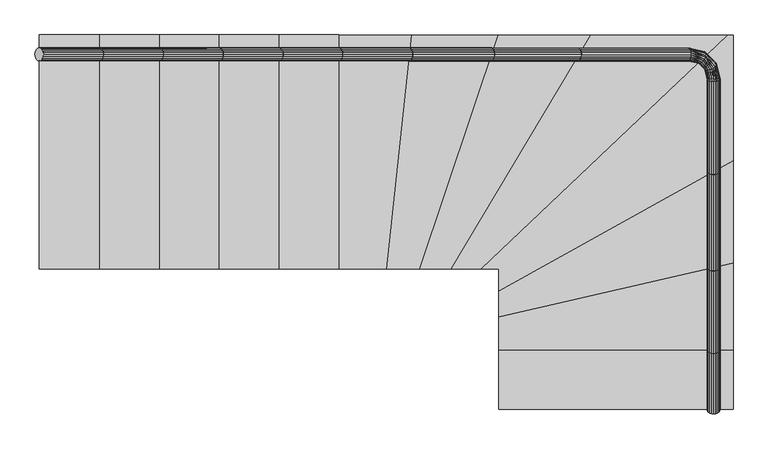
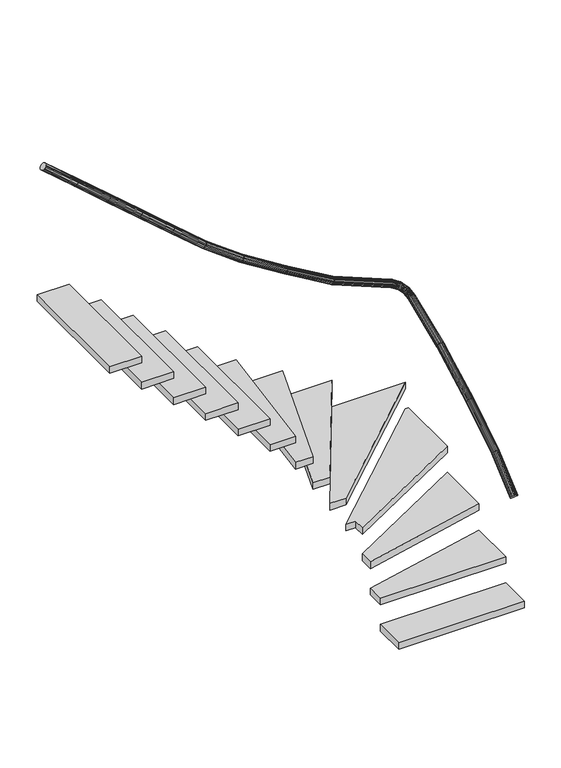
"""IFC4 building model written with IfcOpenShell, lengths in millimetres: stair geometry, 0_3d_modell."""

from ifc_helpers import new_model, si_unit, frame, origin, origin_with_axes, place, context, project, spatial, polyline, outline, extrude, faceted_brep, source, transform, mapped, element, save


def stair_9e6d9002(model_context):
    return source(origin(), model_context, "Body", "SolidModel", [
        extrude(outline(polyline([(1781.5036957, 473.824936), (1781.5036957, 556.9018591), (1711.5036957, 556.9018591), (2658.8332796, 1456.9018591), (2681.5036957, 1456.9018591), (2681.5036957, 973.1970565), (1781.5036957, 473.824936)])), frame((0.0, 0.0, 595.7142857), z_axis=(0.0, 0.0, 1.0), x_axis=(1.0, 0.0, 0.0)), (0.0, 0.0, 1.0), 50.0),
        extrude(outline(polyline([(936.9018591, 556.9018591), (706.9018591, 556.9018591), (706.9018591, 1456.9018591), (936.9018591, 1456.9018591), (936.9018591, 556.9018591)])), frame((0.0, 0.0, 1787.1428571), z_axis=(0.0, 0.0, 1.0), x_axis=(1.0, 0.0, 0.0)), (0.0, 0.0, 1.0), 50.0),
        extrude(outline(polyline([(1.2235871, -7.9923214), (0.0, 0.0), (1.2235871, 7.9923214), (4.7745751, 15.2022987), (10.3053687, 20.9241691), (17.2745751, 24.597836), (25.0, 25.8636953), (32.7254248, 24.597836), (39.6946313, 20.9241691), (45.2254248, 15.2022987), (48.7764129, 7.9923214), (50.0, 0.0), (48.7764129, -7.9923214), (45.2254248, -15.2022986), (39.6946313, -20.9241689), (32.7254248, -24.5978359), (25.0, -25.8636953), (17.2745751, -24.5978359), (10.3053687, -20.9241689), (4.7745751, -15.2022986), (1.2235871, -7.9923214)])), frame((936.9018591, 1406.9018591, 2656.7020937), z_axis=(-0.7569287102857389, 0.0, 0.6534974579485127), x_axis=(0.0, -1.0, 0.0)), (0.0, 0.0, 1.0), 303.8595272),
        extrude(outline(polyline([(1349.1921789, 556.9018591), (1166.9018591, 556.9018591), (1166.9018591, 1456.9018591), (1444.6115394, 1456.9018591), (1349.1921789, 556.9018591)])), frame((0.0, 0.0, 1390.0), z_axis=(0.0, 0.0, 1.0), x_axis=(1.0, 0.0, 0.0)), (0.0, 0.0, 1.0), 50.0),
        extrude(outline(polyline([(1477.0220692, 556.9018591), (1349.1921789, 556.9018591), (1444.6115394, 1456.9018591), (1776.781649, 1456.9018591), (1477.0220692, 556.9018591)])), frame((0.0, 0.0, 1191.4285714), z_axis=(0.0, 0.0, 1.0), x_axis=(1.0, 0.0, 0.0)), (0.0, 0.0, 1.0), 50.0),
        extrude(outline(polyline([(1711.5036957, 556.9018591), (1597.1723093, 556.9018591), (2132.6233472, 1456.9018591), (2658.8332796, 1456.9018591), (1711.5036957, 556.9018591)])), frame((0.0, 0.0, 794.2857143), z_axis=(0.0, 0.0, 1.0), x_axis=(1.0, 0.0, 0.0)), (0.0, 0.0, 1.0), 50.0),
        extrude(outline(polyline([(1.2235871, -7.9923214), (0.0, 0.0), (1.2235871, 7.9923214), (4.7745751, 15.2022986), (10.3053687, 20.924169), (17.2745751, 24.5978359), (25.0, 25.8636953), (32.7254248, 24.5978359), (39.6946313, 20.924169), (45.2254248, 15.2022986), (48.7764129, 7.9923214), (50.0, 0.0), (48.7764129, -7.9923214), (45.2254248, -15.2022986), (39.6946313, -20.924169), (32.7254248, -24.597836), (25.0, -25.8636953), (17.2745751, -24.597836), (10.3053687, -20.924169), (4.7745751, -15.2022986), (1.2235871, -7.9923214)])), frame((246.9018591, 1406.9018591, 3252.4163795), z_axis=(-0.7569287102857456, 0.0, 0.6534974579485049), x_axis=(0.0, -1.0, 0.0)), (0.0, 0.0, 1.0), 303.8595272),
        faceted_brep([(2630.2801086, 935.0213576, 1458.0478269), (2631.5036957, 931.5827131, 1465.2735223), (2630.2801086, 928.1440687, 1472.4992177), (2626.7291206, 925.0420228, 1479.0176117), (2621.198327, 922.5802252, 1484.1906384), (2614.2291206, 920.9996538, 1487.511926), (2606.5036957, 920.4550261, 1488.6563638), (2598.7782709, 920.9996538, 1487.511926), (2591.8090644, 922.5802252, 1484.1906384), (2586.2782709, 925.0420228, 1479.0176117), (2582.7272828, 928.1440687, 1472.4992177), (2581.5036957, 931.5827131, 1465.2735223), (2582.7272828, 935.0213576, 1458.0478269), (2586.2782709, 938.1234035, 1451.529433), (2591.8090644, 940.5852011, 1446.3564062), (2598.7782709, 942.1657724, 1443.0351186), (2606.5036957, 942.7104002, 1441.8906809), (2614.2291206, 942.1657724, 1443.0351186), (2621.198327, 940.5852011, 1446.3564062), (2626.7291206, 938.1234035, 1451.529433), (2630.2801086, 1283.3224302, 1620.3777918), (2631.5036957, 1286.3944101, 1612.9994356), (2630.2801086, 1289.46639, 1605.6210794), (2626.7291206, 1292.2376632, 1598.9649681), (2621.198327, 1294.436958, 1593.6826483), (2614.2291206, 1295.8489921, 1590.2911902), (2606.5036957, 1296.335546, 1589.1225734), (2598.7782709, 1295.8489921, 1590.2911902), (2591.8090644, 1294.436958, 1593.6826483), (2586.2782709, 1292.2376632, 1598.9649681), (2582.7272828, 1289.46639, 1605.6210794), (2581.5036957, 1286.3944101, 1612.9994356), (2582.7272828, 1283.3224302, 1620.3777918), (2586.2782709, 1280.5511571, 1627.0339031), (2591.8090644, 1278.3518623, 1632.3162229), (2598.7782709, 1276.9398281, 1635.707681), (2606.5036957, 1276.4532743, 1636.8762979), (2614.2291206, 1276.9398281, 1635.707681), (2621.198327, 1278.3518623, 1632.3162229), (2626.7291206, 1280.5511571, 1627.0339031)], [[[0, 1, 2, 3, 4, 5, 6, 7, 8, 9, 10, 11, 12, 13, 14, 15, 16, 17, 18, 19]], [[20, 21, 22, 23, 24, 25, 26, 27, 28, 29, 30, 31, 32, 33, 34, 35, 36, 37, 38, 39]], [[2, 1, 21, 20]], [[3, 2, 20, 39]], [[4, 3, 39, 38]], [[5, 4, 38, 37]], [[6, 5, 37, 36]], [[7, 6, 36, 35]], [[8, 7, 35, 34]], [[9, 8, 34, 33]], [[10, 9, 33, 32]], [[11, 10, 32, 31]], [[12, 11, 31, 30]], [[13, 12, 30, 29]], [[14, 13, 29, 28]], [[15, 14, 28, 27]], [[16, 15, 27, 26]], [[17, 16, 26, 25]], [[18, 17, 25, 24]], [[19, 18, 24, 23]], [[0, 19, 23, 22]], [[1, 0, 22, 21]]]),
        extrude(outline(polyline([(1781.5036957, 373.9346688), (1781.5036957, 473.824936), (2681.5036957, 973.1970565), (2681.5036957, 579.8690495), (1781.5036957, 373.9346688)])), frame((0.0, 0.0, 397.1428571), z_axis=(0.0, 0.0, 1.0), x_axis=(1.0, 0.0, 0.0)), (0.0, 0.0, 1.0), 50.0),
        extrude(outline(polyline([(1.2235871, -7.9923214), (0.0, 0.0), (1.2235871, 7.9923214), (4.7745751, 15.2022986), (10.3053687, 20.9241691), (17.2745751, 24.5978359), (25.0, 25.8636953), (32.7254248, 24.5978359), (39.6946313, 20.9241691), (45.2254248, 15.2022986), (48.7764129, 7.9923214), (50.0, 0.0), (48.7764129, -7.9923214), (45.2254248, -15.2022986), (39.6946313, -20.924169), (32.7254248, -24.5978359), (25.0, -25.8636953), (17.2745751, -24.5978359), (10.3053687, -20.924169), (4.7745751, -15.2022986), (1.2235871, -7.9923214)])), frame((476.9018591, 1406.9018591, 3053.8449509), z_axis=(-0.7569287102857636, 0.0, 0.6534974579484839), x_axis=(0.0, -1.0, 0.0)), (0.0, 0.0, 1.0), 303.8595272),
        faceted_brep([(2630.2801086, 566.7337566, 1259.7925307), (2631.5036957, 562.7078511, 1266.7020937), (2630.2801086, 558.6819455, 1273.6116568), (2626.7291206, 555.0501237, 1279.8448636), (2621.198327, 552.1678935, 1284.7915646), (2614.2291206, 550.3173878, 1287.9675421), (2606.5036957, 549.679747, 1289.0619094), (2598.7782709, 550.3173878, 1287.9675421), (2591.8090644, 552.1678935, 1284.7915646), (2586.2782709, 555.0501237, 1279.8448636), (2582.7272828, 558.6819455, 1273.6116568), (2581.5036957, 562.7078511, 1266.7020937), (2582.7272828, 566.7337566, 1259.7925307), (2586.2782709, 570.3655785, 1253.5593239), (2591.8090644, 573.2478087, 1248.6126229), (2598.7782709, 575.0983143, 1245.4366454), (2606.5036957, 575.7359551, 1244.3422781), (2614.2291206, 575.0983143, 1245.4366454), (2621.198327, 573.2478087, 1248.6126229), (2626.7291206, 570.3655785, 1253.5593239), (2630.2801086, 928.1440687, 1472.4992177), (2631.5036957, 931.5827131, 1465.2735223), (2630.2801086, 935.0213576, 1458.0478269), (2626.7291206, 938.1234035, 1451.529433), (2621.198327, 940.5852011, 1446.3564062), (2614.2291206, 942.1657724, 1443.0351186), (2606.5036957, 942.7104002, 1441.8906809), (2598.7782709, 942.1657724, 1443.0351186), (2591.8090644, 940.5852011, 1446.3564062), (2586.2782709, 938.1234035, 1451.529433), (2582.7272828, 935.0213576, 1458.0478269), (2581.5036957, 931.5827131, 1465.2735223), (2582.7272828, 928.1440687, 1472.4992177), (2586.2782709, 925.0420228, 1479.0176117), (2591.8090644, 922.5802252, 1484.1906384), (2598.7782709, 920.9996538, 1487.511926), (2606.5036957, 920.4550261, 1488.6563638), (2614.2291206, 920.9996538, 1487.511926), (2621.198327, 922.5802252, 1484.1906384), (2626.7291206, 925.0420228, 1479.0176117)], [[[0, 1, 2, 3, 4, 5, 6, 7, 8, 9, 10, 11, 12, 13, 14, 15, 16, 17, 18, 19]], [[20, 21, 22, 23, 24, 25, 26, 27, 28, 29, 30, 31, 32, 33, 34, 35, 36, 37, 38, 39]], [[2, 1, 21, 20]], [[3, 2, 20, 39]], [[4, 3, 39, 38]], [[5, 4, 38, 37]], [[6, 5, 37, 36]], [[7, 6, 36, 35]], [[8, 7, 35, 34]], [[9, 8, 34, 33]], [[10, 9, 33, 32]], [[11, 10, 32, 31]], [[12, 11, 31, 30]], [[13, 12, 30, 29]], [[14, 13, 29, 28]], [[15, 14, 28, 27]], [[16, 15, 27, 26]], [[17, 16, 26, 25]], [[18, 17, 25, 24]], [[19, 18, 24, 23]], [[0, 19, 23, 22]], [[1, 0, 22, 21]]]),
        faceted_brep([(2630.2801086, 251.6675536, 1061.6862641), (2631.5036957, 246.9018591, 1068.1306652), (2630.2801086, 242.1361647, 1074.5750662), (2626.7291206, 237.8369696, 1080.3886444), (2621.198327, 234.4251091, 1085.0023262), (2614.2291206, 232.2345598, 1087.9644922), (2606.5036957, 231.4797479, 1088.985185), (2598.7782709, 232.2345598, 1087.9644922), (2591.8090644, 234.4251091, 1085.0023262), (2586.2782709, 237.8369696, 1080.3886444), (2582.7272828, 242.1361647, 1074.5750662), (2581.5036957, 246.9018591, 1068.1306652), (2582.7272828, 251.6675536, 1061.6862641), (2586.2782709, 255.9667486, 1055.872686), (2591.8090644, 259.3786091, 1051.2590042), (2598.7782709, 261.5691584, 1048.2968382), (2606.5036957, 262.3239703, 1047.2761453), (2614.2291206, 261.5691584, 1048.2968382), (2621.198327, 259.3786091, 1051.2590042), (2626.7291206, 255.9667486, 1055.872686), (2630.2801086, 558.6819455, 1273.6116568), (2631.5036957, 562.7078511, 1266.7020937), (2630.2801086, 566.7337566, 1259.7925307), (2626.7291206, 570.3655785, 1253.5593239), (2621.198327, 573.2478087, 1248.6126229), (2614.2291206, 575.0983143, 1245.4366454), (2606.5036957, 575.7359551, 1244.3422781), (2598.7782709, 575.0983143, 1245.4366454), (2591.8090644, 573.2478087, 1248.6126229), (2586.2782709, 570.3655785, 1253.5593239), (2582.7272828, 566.7337566, 1259.7925307), (2581.5036957, 562.7078511, 1266.7020937), (2582.7272828, 558.6819455, 1273.6116568), (2586.2782709, 555.0501237, 1279.8448636), (2591.8090644, 552.1678935, 1284.7915646), (2598.7782709, 550.3173878, 1287.9675421), (2606.5036957, 549.679747, 1289.0619094), (2614.2291206, 550.3173878, 1287.9675421), (2621.198327, 552.1678935, 1284.7915646), (2626.7291206, 555.0501237, 1279.8448636)], [[[0, 1, 2, 3, 4, 5, 6, 7, 8, 9, 10, 11, 12, 13, 14, 15, 16, 17, 18, 19]], [[20, 21, 22, 23, 24, 25, 26, 27, 28, 29, 30, 31, 32, 33, 34, 35, 36, 37, 38, 39]], [[2, 1, 21, 20]], [[3, 2, 20, 39]], [[4, 3, 39, 38]], [[5, 4, 38, 37]], [[6, 5, 37, 36]], [[7, 6, 36, 35]], [[8, 7, 35, 34]], [[9, 8, 34, 33]], [[10, 9, 33, 32]], [[11, 10, 32, 31]], [[12, 11, 31, 30]], [[13, 12, 30, 29]], [[14, 13, 29, 28]], [[15, 14, 28, 27]], [[16, 15, 27, 26]], [[17, 16, 26, 25]], [[18, 17, 25, 24]], [[19, 18, 24, 23]], [[0, 19, 23, 22]], [[1, 0, 22, 21]]]),
        faceted_brep([(2630.2801086, 1289.46639, 1605.6210794), (2631.5036957, 1286.3944101, 1612.9994356), (2630.2801086, 1283.3224302, 1620.3777918), (2626.7291206, 1280.5511571, 1627.0339031), (2621.198327, 1278.3518623, 1632.3162229), (2614.2291206, 1276.9398281, 1635.707681), (2606.5036957, 1276.4532743, 1636.8762979), (2598.7782709, 1276.9398281, 1635.707681), (2591.8090644, 1278.3518623, 1632.3162229), (2586.2782709, 1280.5511571, 1627.0339031), (2582.7272828, 1283.3224302, 1620.3777918), (2581.5036957, 1286.3944101, 1612.9994356), (2582.7272828, 1289.46639, 1605.6210794), (2586.2782709, 1292.2376632, 1598.9649681), (2591.8090644, 1294.436958, 1593.6826483), (2598.7782709, 1295.8489921, 1590.2911902), (2606.5036957, 1296.335546, 1589.1225734), (2614.2291206, 1295.8489921, 1590.2911902), (2621.198327, 1294.436958, 1593.6826483), (2626.7291206, 1292.2376632, 1598.9649681), (2616.4980036, 1348.8501513, 1638.9123688), (2617.3046378, 1344.8271855, 1645.879395), (2615.8855438, 1340.0232633, 1652.1644401), (2612.3796323, 1334.9086261, 1657.1522801), (2607.1300863, 1329.9839302, 1660.3546705), (2600.650768, 1325.7312391, 1661.4581391), (2593.5759183, 1322.5668359, 1660.3546705), (2586.5980727, 1320.8004745, 1657.1522801), (2580.4002713, 1320.6050585, 1652.1644401), (2575.5891981, 1321.9997167, 1645.879395), (2572.6357946, 1324.8479302, 1638.9123688), (2571.8291603, 1328.870896, 1631.9453426), (2573.2482544, 1333.6748181, 1625.6602975), (2576.7541659, 1338.7894554, 1620.6724574), (2582.0037118, 1343.7141513, 1617.470067), (2588.4830301, 1347.9668423, 1616.3665985), (2595.5578799, 1351.1312455, 1617.470067), (2602.5357255, 1352.8976069, 1620.6724574), (2608.7335269, 1353.0930229, 1625.6602975), (2613.5446, 1351.6983647, 1631.9453426), (2573.2894856, 1391.9456089, 1666.2859781), (2576.1190741, 1389.0124344, 1673.2691208), (2577.5017941, 1384.2169558, 1679.5687049), (2577.3022952, 1378.028588, 1684.5680831), (2575.5401057, 1371.0530916, 1687.7778814), (2572.3877211, 1363.9732768, 1688.8839026), (2568.1537188, 1357.4821652, 1687.7778814), (2563.2525523, 1352.215152, 1684.5680831), (2558.163982, 1348.6878091, 1679.5687049), (2553.3861126, 1347.2454175, 1673.2691208), (2549.3866353, 1348.0291684, 1666.2859781), (2546.5570467, 1350.962343, 1659.3028354), (2545.1743267, 1355.7578216, 1653.0032514), (2545.3738257, 1361.9461894, 1648.0038732), (2547.1360151, 1368.9216857, 1644.7940748), (2550.2883997, 1376.0015006, 1643.6880537), (2554.5224021, 1382.4926122, 1644.7940748), (2559.4235686, 1387.7596254, 1648.0038732), (2564.5121389, 1391.2869683, 1653.0032514), (2569.2900082, 1392.7293599, 1659.3028354), (2510.6895066, 1406.9018591, 1691.7803901), (2513.6813624, 1405.678272, 1699.1915978), (2516.3803544, 1402.127284, 1705.8773449), (2518.5222867, 1396.5964904, 1711.1831838), (2519.8974918, 1389.627284, 1714.5897421), (2520.3713552, 1381.9018591, 1715.7635621), (2519.8974918, 1374.1764343, 1714.5897421), (2518.5222867, 1367.2072278, 1711.1831838), (2516.3803544, 1361.6764343, 1705.8773449), (2513.6813624, 1358.1254462, 1699.1915978), (2510.6895066, 1356.9018591, 1691.7803901), (2507.6976509, 1358.1254462, 1684.3691823), (2504.9986588, 1361.6764343, 1677.6834352), (2502.8567266, 1367.2072278, 1672.3775963), (2501.4815215, 1374.1764343, 1668.971038), (2501.0076581, 1381.9018591, 1667.797218), (2501.4815215, 1389.627284, 1668.971038), (2502.8567266, 1396.5964904, 1672.3775963), (2504.9986588, 1402.127284, 1677.6834352), (2507.6976509, 1405.678272, 1684.3691823), (2091.5504886, 1405.678272, 1869.6030507), (2088.0024274, 1406.9018591, 1862.4163795), (2084.4543661, 1405.678272, 1855.2297082), (2081.2536138, 1402.127284, 1848.7465184), (2078.7134824, 1396.5964904, 1843.6014299), (2077.0826177, 1389.627284, 1840.2980797), (2076.52066, 1381.9018591, 1839.1598228), (2077.0826177, 1374.1764343, 1840.2980797), (2078.7134824, 1367.2072278, 1843.6014299), (2081.2536138, 1361.6764343, 1848.7465184), (2084.4543661, 1358.1254462, 1855.2297082), (2088.0024274, 1356.9018591, 1862.4163795), (2091.5504886, 1358.1254462, 1869.6030507), (2094.7512409, 1361.6764343, 1876.0862405), (2097.2913723, 1367.2072278, 1881.231329), (2098.9222371, 1374.1764343, 1884.5346792), (2099.4841948, 1381.9018591, 1885.6729361), (2098.9222371, 1389.627284, 1884.5346792), (2097.2913723, 1396.5964904, 1881.231329), (2094.7512409, 1402.127284, 1876.0862405)], [[[0, 1, 2, 3, 4, 5, 6, 7, 8, 9, 10, 11, 12, 13, 14, 15, 16, 17, 18, 19]], [[2, 1, 20]], [[21, 2, 20]], [[3, 2, 21]], [[22, 3, 21]], [[4, 3, 22]], [[23, 4, 22]], [[5, 4, 23]], [[24, 5, 23]], [[6, 5, 24]], [[25, 6, 24]], [[7, 6, 25]], [[26, 7, 25]], [[8, 7, 26]], [[27, 8, 26]], [[9, 8, 27]], [[28, 9, 27]], [[10, 9, 28]], [[29, 10, 28]], [[11, 10, 29]], [[30, 11, 29]], [[12, 11, 30]], [[31, 12, 30]], [[13, 12, 31]], [[32, 13, 31]], [[14, 13, 32]], [[33, 14, 32]], [[15, 14, 33]], [[34, 15, 33]], [[16, 15, 34]], [[35, 16, 34]], [[17, 16, 35]], [[36, 17, 35]], [[18, 17, 36]], [[37, 18, 36]], [[19, 18, 37]], [[38, 19, 37]], [[0, 19, 38]], [[39, 0, 38]], [[1, 0, 39]], [[20, 1, 39]], [[21, 20, 40]], [[41, 21, 40]], [[22, 21, 41]], [[42, 22, 41]], [[23, 22, 42]], [[43, 23, 42]], [[24, 23, 43]], [[44, 24, 43]], [[25, 24, 44]], [[45, 25, 44]], [[26, 25, 45]], [[46, 26, 45]], [[27, 26, 46]], [[47, 27, 46]], [[28, 27, 47]], [[48, 28, 47]], [[29, 28, 48]], [[49, 29, 48]], [[30, 29, 49]], [[50, 30, 49]], [[31, 30, 50]], [[51, 31, 50]], [[32, 31, 51]], [[52, 32, 51]], [[33, 32, 52]], [[53, 33, 52]], [[34, 33, 53]], [[54, 34, 53]], [[35, 34, 54]], [[55, 35, 54]], [[36, 35, 55]], [[56, 36, 55]], [[37, 36, 56]], [[57, 37, 56]], [[38, 37, 57]], [[58, 38, 57]], [[39, 38, 58]], [[59, 39, 58]], [[20, 39, 59]], [[40, 20, 59]], [[41, 40, 60]], [[61, 41, 60]], [[42, 41, 61]], [[62, 42, 61]], [[43, 42, 62]], [[63, 43, 62]], [[44, 43, 63]], [[64, 44, 63]], [[45, 44, 64]], [[65, 45, 64]], [[46, 45, 65]], [[66, 46, 65]], [[47, 46, 66]], [[67, 47, 66]], [[48, 47, 67]], [[68, 48, 67]], [[49, 48, 68]], [[69, 49, 68]], [[50, 49, 69]], [[70, 50, 69]], [[51, 50, 70]], [[71, 51, 70]], [[52, 51, 71]], [[72, 52, 71]], [[53, 52, 72]], [[73, 53, 72]], [[54, 53, 73]], [[74, 54, 73]], [[55, 54, 74]], [[75, 55, 74]], [[56, 55, 75]], [[76, 56, 75]], [[57, 56, 76]], [[77, 57, 76]], [[58, 57, 77]], [[78, 58, 77]], [[59, 58, 78]], [[79, 59, 78]], [[40, 59, 79]], [[60, 40, 79]], [[80, 81, 82, 83, 84, 85, 86, 87, 88, 89, 90, 91, 92, 93, 94, 95, 96, 97, 98, 99]], [[61, 60, 81, 80]], [[62, 61, 80, 99]], [[63, 62, 99, 98]], [[64, 63, 98, 97]], [[65, 64, 97, 96]], [[66, 65, 96, 95]], [[67, 66, 95, 94]], [[68, 67, 94, 93]], [[69, 68, 93, 92]], [[70, 69, 92, 91]], [[71, 70, 91, 90]], [[72, 71, 90, 89]], [[73, 72, 89, 88]], [[74, 73, 88, 87]], [[75, 74, 87, 86]], [[76, 75, 86, 85]], [[77, 76, 85, 84]], [[78, 77, 84, 83]], [[79, 78, 83, 82]], [[60, 79, 82, 81]]]),
        extrude(outline(polyline([(1781.5036957, 16.9018591), (1781.5036957, 246.9018591), (2681.5036957, 246.9018591), (2681.5036957, 16.9018591), (1781.5036957, 16.9018591)])), origin_with_axes(), (0.0, 0.0, 1.0), 50.0),
        extrude(outline(polyline([(246.9018591, 556.9018591), (16.9018591, 556.9018591), (16.9018591, 1456.9018591), (246.9018591, 1456.9018591), (246.9018591, 556.9018591)])), frame((0.0, 0.0, 2382.8571429), z_axis=(0.0, 0.0, 1.0), x_axis=(1.0, 0.0, 0.0)), (0.0, 0.0, 1.0), 50.0),
        extrude(outline(polyline([(1.2235871, -7.9923214), (0.0, 0.0), (1.2235871, 7.9923214), (4.7745751, 15.2022986), (10.3053687, 20.9241691), (17.2745751, 24.5978359), (25.0, 25.8636953), (32.7254248, 24.5978359), (39.6946313, 20.9241691), (45.2254248, 15.2022986), (48.7764129, 7.9923214), (50.0, 0.0), (48.7764129, -7.9923214), (45.2254248, -15.2022986), (39.6946313, -20.9241689), (32.7254248, -24.5978359), (25.0, -25.8636953), (17.2745751, -24.5978359), (10.3053687, -20.9241689), (4.7745751, -15.2022986), (1.2235871, -7.9923214)])), frame((706.9018591, 1406.9018591, 2855.2735223), z_axis=(-0.756928710285736, 0.0, 0.6534974579485159), x_axis=(0.0, -1.0, 0.0)), (0.0, 0.0, 1.0), 303.8595272),
        faceted_brep([(1747.6382113, 1405.678272, 2054.1646194), (1751.801684, 1406.9018591, 2060.987808), (1755.9651567, 1405.678272, 2067.8109967), (1759.7210797, 1402.127284, 2073.966284), (1762.701797, 1396.5964904, 2078.8511477), (1764.6155354, 1389.627284, 2081.9874233), (1765.2749647, 1381.9018591, 2083.0681102), (1764.6155354, 1374.1764343, 2081.9874233), (1762.701797, 1367.2072278, 2078.8511477), (1759.7210797, 1361.6764343, 2073.966284), (1755.9651567, 1358.1254462, 2067.8109967), (1751.801684, 1356.9018591, 2060.987808), (1747.6382113, 1358.1254462, 2054.1646194), (1743.8822884, 1361.6764343, 2048.009332), (1740.901571, 1367.2072278, 2043.1244683), (1738.9878327, 1374.1764343, 2039.9881928), (1738.3284034, 1381.9018591, 2038.9075058), (1738.9878327, 1389.627284, 2039.9881928), (1740.901571, 1396.5964904, 2043.1244683), (1743.8822884, 1402.127284, 2048.009332), (1441.1651504, 1405.678272, 2266.1670868), (1436.659926, 1406.9018591, 2259.5592366), (1432.1547015, 1405.678272, 2252.9513864), (1428.0904799, 1402.127284, 2246.9903587), (1424.8650953, 1396.5964904, 2242.2596602), (1422.7942709, 1389.627284, 2239.2223649), (1422.0807134, 1381.9018591, 2238.1757842), (1422.7942709, 1374.1764343, 2239.2223649), (1424.8650953, 1367.2072278, 2242.2596602), (1428.0904799, 1361.6764343, 2246.9903587), (1432.1547015, 1358.1254462, 2252.9513864), (1436.659926, 1356.9018591, 2259.5592366), (1441.1651504, 1358.1254462, 2266.1670868), (1445.2293721, 1361.6764343, 2272.1281145), (1448.4547567, 1367.2072278, 2276.858813), (1450.5255811, 1374.1764343, 2279.8961083), (1451.2391385, 1381.9018591, 2280.942689), (1450.5255811, 1389.627284, 2279.8961083), (1448.4547567, 1396.5964904, 2276.858813), (1445.2293721, 1402.127284, 2272.1281145)], [[[0, 1, 2, 3, 4, 5, 6, 7, 8, 9, 10, 11, 12, 13, 14, 15, 16, 17, 18, 19]], [[20, 21, 22, 23, 24, 25, 26, 27, 28, 29, 30, 31, 32, 33, 34, 35, 36, 37, 38, 39]], [[2, 1, 21, 20]], [[3, 2, 20, 39]], [[4, 3, 39, 38]], [[5, 4, 38, 37]], [[6, 5, 37, 36]], [[7, 6, 36, 35]], [[8, 7, 35, 34]], [[9, 8, 34, 33]], [[10, 9, 33, 32]], [[11, 10, 32, 31]], [[12, 11, 31, 30]], [[13, 12, 30, 29]], [[14, 13, 29, 28]], [[15, 14, 28, 27]], [[16, 15, 27, 26]], [[17, 16, 26, 25]], [[18, 17, 25, 24]], [[19, 18, 24, 23]], [[0, 19, 23, 22]], [[1, 0, 22, 21]]]),
        extrude(outline(polyline([(1597.1723093, 556.9018591), (1477.0220692, 556.9018591), (1776.781649, 1456.9018591), (2132.6233472, 1456.9018591), (1597.1723093, 556.9018591)])), frame((0.0, 0.0, 992.8571429), z_axis=(0.0, 0.0, 1.0), x_axis=(1.0, 0.0, 0.0)), (0.0, 0.0, 1.0), 50.0),
        extrude(outline(polyline([(1166.9018591, 556.9018591), (936.9018591, 556.9018591), (936.9018591, 1456.9018591), (1166.9018591, 1456.9018591), (1166.9018591, 556.9018591)])), frame((0.0, 0.0, 1588.5714286), z_axis=(0.0, 0.0, 1.0), x_axis=(1.0, 0.0, 0.0)), (0.0, 0.0, 1.0), 50.0),
        faceted_brep([(2630.2801086, 22.1248208, 863.5096191), (2631.5036957, 16.9018591, 869.5592366), (2630.2801086, 11.6788974, 875.6088541), (2626.7291206, 6.9671956, 881.0662929), (2621.198327, 3.2279679, 885.3973409), (2614.2291206, 0.8272359, 888.1780448), (2606.5036957, 0.0, 889.1362101), (2598.7782709, 0.8272359, 888.1780448), (2591.8090644, 3.2279679, 885.3973409), (2586.2782709, 6.9671956, 881.0662929), (2582.7272828, 11.6788974, 875.6088541), (2581.5036957, 16.9018591, 869.5592366), (2582.7272828, 22.1248208, 863.5096191), (2586.2782709, 26.8365226, 858.0521803), (2591.8090644, 30.5757504, 853.7211323), (2598.7782709, 32.9764824, 850.9404284), (2606.5036957, 33.8037182, 849.9822631), (2614.2291206, 32.9764824, 850.9404284), (2621.198327, 30.5757504, 853.7211323), (2626.7291206, 26.8365226, 858.0521803), (2630.2801086, 242.1361647, 1074.5750662), (2631.5036957, 246.9018591, 1068.1306652), (2630.2801086, 251.6675536, 1061.6862641), (2626.7291206, 255.9667486, 1055.872686), (2621.198327, 259.3786091, 1051.2590042), (2614.2291206, 261.5691584, 1048.2968382), (2606.5036957, 262.3239703, 1047.2761453), (2598.7782709, 261.5691584, 1048.2968382), (2591.8090644, 259.3786091, 1051.2590042), (2586.2782709, 255.9667486, 1055.872686), (2582.7272828, 251.6675536, 1061.6862641), (2581.5036957, 246.9018591, 1068.1306652), (2582.7272828, 242.1361647, 1074.5750662), (2586.2782709, 237.8369696, 1080.3886444), (2591.8090644, 234.4251091, 1085.0023262), (2598.7782709, 232.2345598, 1087.9644922), (2606.5036957, 231.4797479, 1088.985185), (2614.2291206, 232.2345598, 1087.9644922), (2621.198327, 234.4251091, 1085.0023262), (2626.7291206, 237.8369696, 1080.3886444)], [[[0, 1, 2, 3, 4, 5, 6, 7, 8, 9, 10, 11, 12, 13, 14, 15, 16, 17, 18, 19]], [[20, 21, 22, 23, 24, 25, 26, 27, 28, 29, 30, 31, 32, 33, 34, 35, 36, 37, 38, 39]], [[2, 1, 21, 20]], [[3, 2, 20, 39]], [[4, 3, 39, 38]], [[5, 4, 38, 37]], [[6, 5, 37, 36]], [[7, 6, 36, 35]], [[8, 7, 35, 34]], [[9, 8, 34, 33]], [[10, 9, 33, 32]], [[11, 10, 32, 31]], [[12, 11, 31, 30]], [[13, 12, 30, 29]], [[14, 13, 29, 28]], [[15, 14, 28, 27]], [[16, 15, 27, 26]], [[17, 16, 26, 25]], [[18, 17, 25, 24]], [[19, 18, 24, 23]], [[0, 19, 23, 22]], [[1, 0, 22, 21]]]),
        faceted_brep([(1432.1547015, 1405.678272, 2252.9513864), (1436.659926, 1406.9018591, 2259.5592366), (1441.1651504, 1405.678272, 2266.1670868), (1445.2293721, 1402.127284, 2272.1281145), (1448.4547567, 1396.5964904, 2276.858813), (1450.5255811, 1389.627284, 2279.8961083), (1451.2391385, 1381.9018591, 2280.942689), (1450.5255811, 1374.1764343, 2279.8961083), (1448.4547567, 1367.2072278, 2276.858813), (1445.2293721, 1361.6764343, 2272.1281145), (1441.1651504, 1358.1254462, 2266.1670868), (1436.659926, 1356.9018591, 2259.5592366), (1432.1547015, 1358.1254462, 2252.9513864), (1428.0904799, 1361.6764343, 2246.9903587), (1424.8650953, 1367.2072278, 2242.2596602), (1422.7942709, 1374.1764343, 2239.2223649), (1422.0807134, 1381.9018591, 2238.1757842), (1422.7942709, 1389.627284, 2239.2223649), (1424.8650953, 1396.5964904, 2242.2596602), (1428.0904799, 1402.127284, 2246.9903587), (1171.8898438, 1405.678272, 2464.383151), (1166.9018591, 1406.9018591, 2458.1306652), (1161.9138744, 1405.678272, 2451.8781793), (1157.4141484, 1402.127284, 2446.2377304), (1153.8431456, 1396.5964904, 2441.7614447), (1151.5504206, 1389.627284, 2438.8874925), (1150.7604015, 1381.9018591, 2437.897196), (1151.5504206, 1374.1764343, 2438.8874925), (1153.8431456, 1367.2072278, 2441.7614447), (1157.4141484, 1361.6764343, 2446.2377304), (1161.9138744, 1358.1254462, 2451.8781793), (1166.9018591, 1356.9018591, 2458.1306652), (1171.8898438, 1358.1254462, 2464.383151), (1176.3895699, 1361.6764343, 2470.0236), (1179.9605727, 1367.2072278, 2474.4998856), (1182.2532976, 1374.1764343, 2477.3738379), (1183.0433167, 1381.9018591, 2478.3641344), (1182.2532976, 1389.627284, 2477.3738379), (1179.9605727, 1396.5964904, 2474.4998856), (1176.3895699, 1402.127284, 2470.0236)], [[[0, 1, 2, 3, 4, 5, 6, 7, 8, 9, 10, 11, 12, 13, 14, 15, 16, 17, 18, 19]], [[20, 21, 22, 23, 24, 25, 26, 27, 28, 29, 30, 31, 32, 33, 34, 35, 36, 37, 38, 39]], [[2, 1, 21, 20]], [[3, 2, 20, 39]], [[4, 3, 39, 38]], [[5, 4, 38, 37]], [[6, 5, 37, 36]], [[7, 6, 36, 35]], [[8, 7, 35, 34]], [[9, 8, 34, 33]], [[10, 9, 33, 32]], [[11, 10, 32, 31]], [[12, 11, 31, 30]], [[13, 12, 30, 29]], [[14, 13, 29, 28]], [[15, 14, 28, 27]], [[16, 15, 27, 26]], [[17, 16, 26, 25]], [[18, 17, 25, 24]], [[19, 18, 24, 23]], [[0, 19, 23, 22]], [[1, 0, 22, 21]]]),
        extrude(outline(polyline([(476.9018591, 556.9018591), (246.9018591, 556.9018591), (246.9018591, 1456.9018591), (476.9018591, 1456.9018591), (476.9018591, 556.9018591)])), frame((0.0, 0.0, 2184.2857143), z_axis=(0.0, 0.0, 1.0), x_axis=(1.0, 0.0, 0.0)), (0.0, 0.0, 1.0), 50.0),
        faceted_brep([(2084.4543661, 1405.678272, 1855.2297082), (2088.0024274, 1406.9018591, 1862.4163795), (2091.5504886, 1405.678272, 1869.6030507), (2094.7512409, 1402.127284, 1876.0862405), (2097.2913723, 1396.5964904, 1881.231329), (2098.9222371, 1389.627284, 1884.5346792), (2099.4841948, 1381.9018591, 1885.6729361), (2098.9222371, 1374.1764343, 1884.5346792), (2097.2913723, 1367.2072278, 1881.231329), (2094.7512409, 1361.6764343, 1876.0862405), (2091.5504886, 1358.1254462, 1869.6030507), (2088.0024274, 1356.9018591, 1862.4163795), (2084.4543661, 1358.1254462, 1855.2297082), (2081.2536138, 1361.6764343, 1848.7465184), (2078.7134824, 1367.2072278, 1843.6014299), (2077.0826177, 1374.1764343, 1840.2980797), (2076.52066, 1381.9018591, 1839.1598228), (2077.0826177, 1389.627284, 1840.2980797), (2078.7134824, 1396.5964904, 1843.6014299), (2081.2536138, 1402.127284, 1848.7465184), (1755.9651567, 1405.678272, 2067.8109967), (1751.801684, 1406.9018591, 2060.987808), (1747.6382113, 1405.678272, 2054.1646194), (1743.8822884, 1402.127284, 2048.009332), (1740.901571, 1396.5964904, 2043.1244683), (1738.9878327, 1389.627284, 2039.9881928), (1738.3284034, 1381.9018591, 2038.9075058), (1738.9878327, 1374.1764343, 2039.9881928), (1740.901571, 1367.2072278, 2043.1244683), (1743.8822884, 1361.6764343, 2048.009332), (1747.6382113, 1358.1254462, 2054.1646194), (1751.801684, 1356.9018591, 2060.987808), (1755.9651567, 1358.1254462, 2067.8109967), (1759.7210797, 1361.6764343, 2073.966284), (1762.701797, 1367.2072278, 2078.8511477), (1764.6155354, 1374.1764343, 2081.9874233), (1765.2749647, 1381.9018591, 2083.0681102), (1764.6155354, 1389.627284, 2081.9874233), (1762.701797, 1396.5964904, 2078.8511477), (1759.7210797, 1402.127284, 2073.966284)], [[[0, 1, 2, 3, 4, 5, 6, 7, 8, 9, 10, 11, 12, 13, 14, 15, 16, 17, 18, 19]], [[20, 21, 22, 23, 24, 25, 26, 27, 28, 29, 30, 31, 32, 33, 34, 35, 36, 37, 38, 39]], [[2, 1, 21, 20]], [[3, 2, 20, 39]], [[4, 3, 39, 38]], [[5, 4, 38, 37]], [[6, 5, 37, 36]], [[7, 6, 36, 35]], [[8, 7, 35, 34]], [[9, 8, 34, 33]], [[10, 9, 33, 32]], [[11, 10, 32, 31]], [[12, 11, 31, 30]], [[13, 12, 30, 29]], [[14, 13, 29, 28]], [[15, 14, 28, 27]], [[16, 15, 27, 26]], [[17, 16, 26, 25]], [[18, 17, 25, 24]], [[19, 18, 24, 23]], [[0, 19, 23, 22]], [[1, 0, 22, 21]]]),
        extrude(outline(polyline([(706.9018591, 556.9018591), (476.9018591, 556.9018591), (476.9018591, 1456.9018591), (706.9018591, 1456.9018591), (706.9018591, 556.9018591)])), frame((0.0, 0.0, 1985.7142857), z_axis=(0.0, 0.0, 1.0), x_axis=(1.0, 0.0, 0.0)), (0.0, 0.0, 1.0), 50.0),
        faceted_brep([(1161.9138744, 1405.678272, 2451.8781793), (1166.9018591, 1406.9018591, 2458.1306652), (1171.8898438, 1405.678272, 2464.383151), (1176.3895699, 1402.127284, 2470.0236), (1179.9605727, 1396.5964904, 2474.4998856), (1182.2532976, 1389.627284, 2477.3738379), (1183.0433167, 1381.9018591, 2478.3641344), (1182.2532976, 1374.1764343, 2477.3738379), (1179.9605727, 1367.2072278, 2474.4998856), (1176.3895699, 1361.6764343, 2470.0236), (1171.8898438, 1358.1254462, 2464.383151), (1166.9018591, 1356.9018591, 2458.1306652), (1161.9138744, 1358.1254462, 2451.8781793), (1157.4141484, 1361.6764343, 2446.2377304), (1153.8431456, 1367.2072278, 2441.7614447), (1151.5504206, 1374.1764343, 2438.8874925), (1150.7604015, 1381.9018591, 2437.897196), (1151.5504206, 1389.627284, 2438.8874925), (1153.8431456, 1396.5964904, 2441.7614447), (1157.4141484, 1402.127284, 2446.2377304), (942.1248208, 1405.678272, 2662.7517113), (936.9018591, 1406.9018591, 2656.7020937), (931.6788974, 1405.678272, 2650.6524762), (926.9671956, 1402.127284, 2645.1950374), (923.2279679, 1396.5964904, 2640.8639895), (920.8272359, 1389.627284, 2638.0832855), (920.0, 1381.9018591, 2637.1251202), (920.8272359, 1374.1764343, 2638.0832855), (923.2279679, 1367.2072278, 2640.8639895), (926.9671956, 1361.6764343, 2645.1950374), (931.6788974, 1358.1254462, 2650.6524762), (936.9018591, 1356.9018591, 2656.7020937), (942.1248208, 1358.1254462, 2662.7517113), (946.8365226, 1361.6764343, 2668.2091501), (950.5757504, 1367.2072278, 2672.540198), (952.9764824, 1374.1764343, 2675.320902), (953.8037182, 1381.9018591, 2676.2790673), (952.9764824, 1389.627284, 2675.320902), (950.5757504, 1396.5964904, 2672.540198), (946.8365226, 1402.127284, 2668.2091501)], [[[0, 1, 2, 3, 4, 5, 6, 7, 8, 9, 10, 11, 12, 13, 14, 15, 16, 17, 18, 19]], [[20, 21, 22, 23, 24, 25, 26, 27, 28, 29, 30, 31, 32, 33, 34, 35, 36, 37, 38, 39]], [[2, 1, 21, 20]], [[3, 2, 20, 39]], [[4, 3, 39, 38]], [[5, 4, 38, 37]], [[6, 5, 37, 36]], [[7, 6, 36, 35]], [[8, 7, 35, 34]], [[9, 8, 34, 33]], [[10, 9, 33, 32]], [[11, 10, 32, 31]], [[12, 11, 31, 30]], [[13, 12, 30, 29]], [[14, 13, 29, 28]], [[15, 14, 28, 27]], [[16, 15, 27, 26]], [[17, 16, 26, 25]], [[18, 17, 25, 24]], [[19, 18, 24, 23]], [[0, 19, 23, 22]], [[1, 0, 22, 21]]]),
        extrude(outline(polyline([(1781.5036957, 246.9018591), (1781.5036957, 373.9346688), (2681.5036957, 579.8690495), (2681.5036957, 246.9018591), (1781.5036957, 246.9018591)])), frame((0.0, 0.0, 198.5714286), z_axis=(0.0, 0.0, 1.0), x_axis=(1.0, 0.0, 0.0)), (0.0, 0.0, 1.0), 50.0),
    ])


if __name__ == "__main__":
    model = new_model("IFC4")
    model_context = context("Model", 3, world=origin())
    ifc_project = project(units=[si_unit("LENGTHUNIT", "METRE", prefix="MILLI")], contexts=[model_context])
    site = spatial("IfcSite", under=ifc_project)
    building = spatial("IfcBuilding", under=site)
    placement = place(None, origin())
    stair_shape = stair_9e6d9002(model_context)
    element("IfcStair", 1, ObjectType="0_3d_modell", at=placement, inside=building, context=model_context, shape_type="MappedRepresentation", body=[
        mapped(stair_shape, transform((0.0, 0.0, 0.0), x_axis=(1.0, 0.0, 0.0), y_axis=(0.0, 1.0, 0.0), z_axis=(0.0, 0.0, 1.0))),
    ])
    save(model, "model.ifc")

# Revit data of these elements
# Element 1 (IfcStair, "0_3d_modell")
#   Materials on its faces: "*1", "weiss"
# Materials
#   "*1": class "Unassigned", colour RGB 175 175 175, transparency 0
#   "weiss": class "Unassigned", colour RGB 255 255 255, transparency 0
